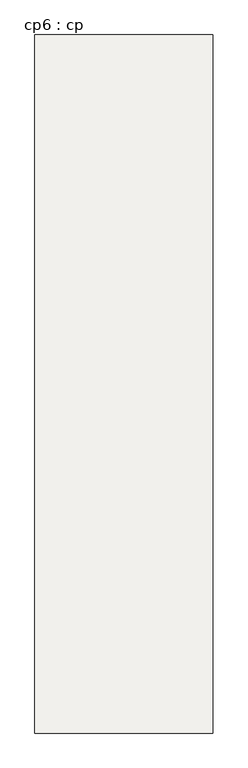
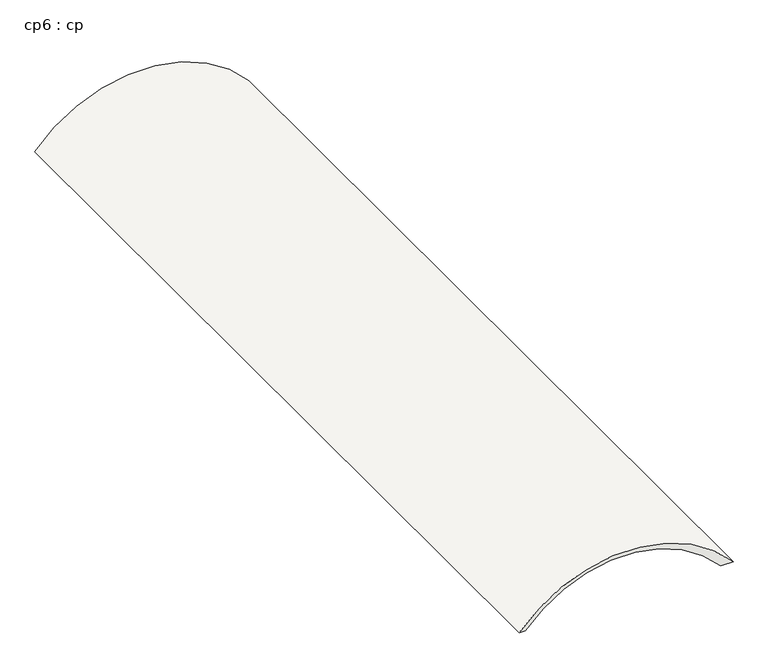
"""IFC4 building model written with IfcOpenShell, lengths in millimetres: slab geometry, cp6 : cp."""

from ifc_helpers import new_model, si_unit, point, frame, frame_2d, origin, place, context, project, spatial, polyline, circle_curve, trimmed, segment, composite_curve, outline, extrude, source, transform, mapped, element, save


def cp6_cp_d200dcca(model_context):
    return source(origin(), model_context, "Body", "SweptSolid", [
        extrude(outline(composite_curve([segment(polyline([(14620.0, 50183.2245511), (14620.0, 50483.2245511)]), True, "CONTINUOUS"), segment(trimmed(circle_curve(frame_2d((12402.7966102, 47908.2245512)), 3398.0311757), [point((14620.0, 50483.2245511))], [point((14620.0, 45333.2245512))], False, "CARTESIAN"), True, "CONTINUOUS"), segment(polyline([(14620.0, 45333.2245512), (14620.0, 45483.2245512)]), True, "CONTINUOUS"), segment(trimmed(circle_curve(frame_2d((12608.2612414, 47833.2245512)), 3093.4758497), [point((14620.0, 45483.2245512))], [point((14620.0, 50183.2245511))], True, "CARTESIAN"), True, "CONTINUOUS")], self_intersect=False)), frame((0.0, -100.2551788, 0.0), z_axis=(0.0, 1.0, 0.0), x_axis=(0.0, 0.0, 1.0)), (0.0, 0.0, 1.0), 20199.9999981),
    ])


if __name__ == "__main__":
    model = new_model("IFC4")
    model_context = context("Model", 3, world=origin())
    ifc_project = project(units=[si_unit("LENGTHUNIT", "METRE", prefix="MILLI")], contexts=[model_context])
    site = spatial("IfcSite", under=ifc_project)
    building = spatial("IfcBuilding", under=site)
    placement = place(None, origin())
    cp6_cp_shape = cp6_cp_d200dcca(model_context)
    element("IfcSlab", 1, ObjectType="cp6 : cp", at=placement, inside=building, context=model_context, shape_type="MappedRepresentation", body=[
        mapped(cp6_cp_shape, transform((0.0, 0.0, 0.0), x_axis=(1.0, 0.0, 0.0), y_axis=(0.0, 1.0, 0.0), z_axis=(0.0, 0.0, 1.0))),
    ])
    save(model, "model.ifc")

# Revit data of these elements
# Type "cp6 : cp"
#   Structural Material = Concrete, RC
# Element 1 (IfcSlab, "cp6 : cp")
#   Materials on its faces: "Concrete, RC"
# Materials
#   "Concrete, RC": class "Concrete", colour RGB 128 128 128, transparency 0, Description = "Cast-in-place concrete", Cost = 0
